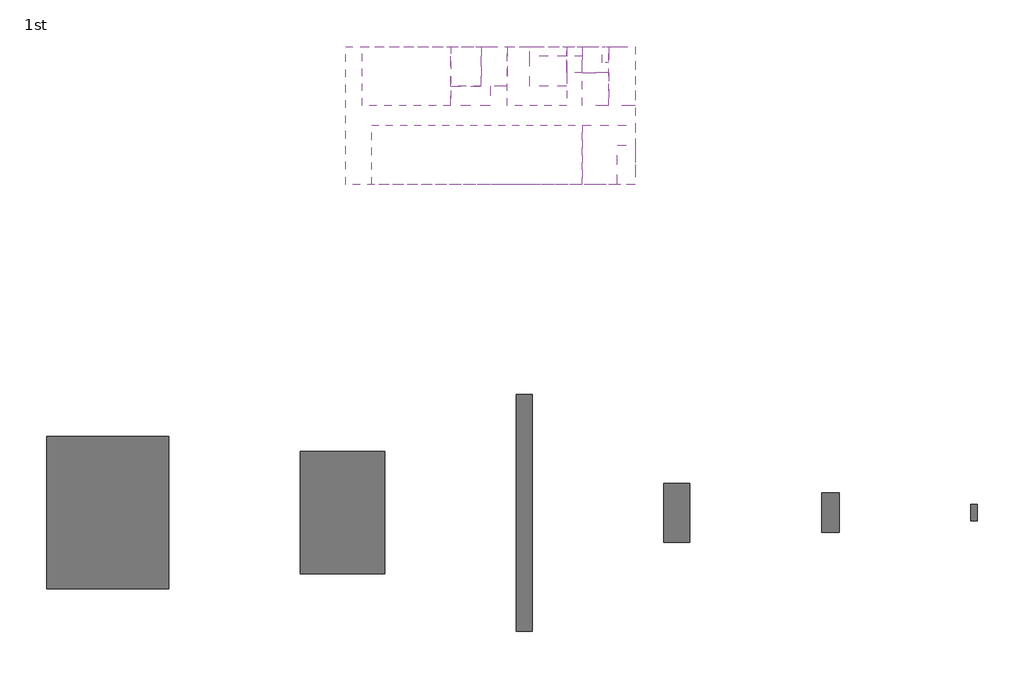
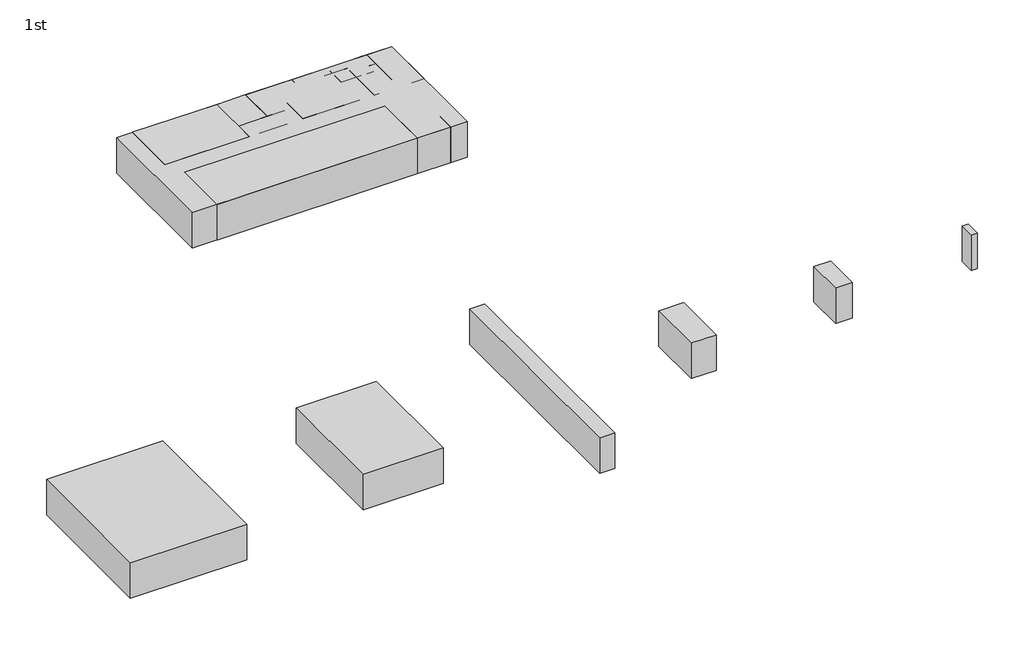
# One storey: 23 proxies.
"""IFC4 building model written with IfcOpenShell, lengths in millimetres."""

import ifcopenshell
import ifcopenshell.guid

model = None  # the IFC model being written
_history = None  # IfcOwnerHistory: only IFC2X3 demands one
_inside = {}  # id of a spatial element -> (the spatial element, [elements in it])
_under = {}  # id of a project, library or spatial element -> (it, [spatial elements below it])
_declared = {}  # id of a project -> (the project, [libraries it declares])
_typed = {}  # id of a type object -> (the type object, [elements of that type])
_made_of = {}  # id of a material, layer set ... -> (it, [elements and type objects made of it])


def new_model(schema):
    """Start an empty IFC model of exactly this schema.

    Asked for "IFC4X3", IfcOpenShell would pick the latest addendum, in which some entities
    have other attributes; the version numbers below select the first issue.
    IFC2X3 requires an IfcOwnerHistory on every rooted entity: one is made here for all.
    """
    global model, _history
    if schema == "IFC4X3":
        model = ifcopenshell.file(schema_version=(4, 3, 0, 0))
    else:
        model = ifcopenshell.file(schema=schema)
    _inside.clear()
    _under.clear()
    _declared.clear()
    _typed.clear()
    _made_of.clear()
    _history = None
    if model.schema == "IFC2X3":
        org = make("IfcOrganization", Name="unknown")
        user = make(
            "IfcPersonAndOrganization",
            ThePerson=make("IfcPerson", FamilyName="unknown"),
            TheOrganization=org,
        )
        app = make(
            "IfcApplication",
            ApplicationDeveloper=org,
            Version="unknown",
            ApplicationFullName="unknown",
            ApplicationIdentifier="unknown",
        )
        _history = make(
            "IfcOwnerHistory",
            OwningUser=user,
            OwningApplication=app,
            ChangeAction="ADDED",
            CreationDate=0,
        )
    return model


def make(cls, **values):
    """One entity of the class cls with the attributes given. An attribute that is None is left unset."""
    return model.create_entity(
        cls, **{name: value for name, value in values.items() if value is not None}
    )


def rooted(cls, **values):
    """An entity with a GlobalId (a new one), such as an element, a storey or a relation."""
    return make(cls, GlobalId=ifcopenshell.guid.new(), OwnerHistory=_history, **values)


def si_unit(unit_type, name, prefix=None):
    """IfcSIUnit, for example si_unit("LENGTHUNIT", "METRE", prefix="MILLI")."""
    return make("IfcSIUnit", UnitType=unit_type, Prefix=prefix, Name=name)


def assignment(units):
    """IfcUnitAssignment: the units of a project."""
    return None if units is None else make("IfcUnitAssignment", Units=units)


def point(xyz):
    """IfcCartesianPoint."""
    return None if xyz is None else make("IfcCartesianPoint", Coordinates=xyz)


def direction(xyz):
    """IfcDirection."""
    return None if xyz is None else make("IfcDirection", DirectionRatios=xyz)


def frame(location, z_axis=None, x_axis=None):
    """IfcAxis2Placement3D, a coordinate frame: its origin and axes. An axis left out is left unset."""
    return make(
        "IfcAxis2Placement3D",
        Location=point(location),
        Axis=direction(z_axis),
        RefDirection=direction(x_axis),
    )


def origin():
    """The frame at (0, 0, 0) with its axes left unset."""
    return frame((0.0, 0.0, 0.0))


def origin_with_axes():
    """The frame at (0, 0, 0) with the z axis (0, 0, 1) and the x axis (1, 0, 0) written out."""
    return frame((0.0, 0.0, 0.0), z_axis=(0.0, 0.0, 1.0), x_axis=(1.0, 0.0, 0.0))


def place(relative_to, where):
    """IfcLocalPlacement: puts the frame where relative to a parent placement (None: the world)."""
    return make(
        "IfcLocalPlacement", PlacementRelTo=relative_to, RelativePlacement=where
    )


def context(
    kind, dimensions, precision=None, world=None, true_north=None, identifier=None
):
    """IfcGeometricRepresentationContext, for example the 3D "Model" context."""
    return make(
        "IfcGeometricRepresentationContext",
        ContextIdentifier=identifier,
        ContextType=kind,
        CoordinateSpaceDimension=dimensions,
        Precision=precision,
        WorldCoordinateSystem=world,
        TrueNorth=true_north,
    )


def project(units=None, contexts=None):
    """IfcProject with its units and contexts."""
    return rooted(
        "IfcProject",
        Name="project",
        RepresentationContexts=contexts,
        UnitsInContext=assignment(units),
    )


def spatial(cls, under=None, at=None, **own):
    """A site, building, storey or space (cls), placed at a placement, below another one or the project."""
    s = rooted(cls, ObjectPlacement=at, **own)
    if under is not None:
        _under.setdefault(under.id(), (under, []))[1].append(s)
    return s


def polyline(points):
    """IfcPolyline through the points."""
    return make("IfcPolyline", Points=[point(p) for p in points])


def outline(outer, holes=None, kind="AREA"):
    """IfcArbitraryClosedProfileDef: a profile drawn as a closed curve; with holes, ...WithVoids."""
    if holes is None:
        return make("IfcArbitraryClosedProfileDef", ProfileType=kind, OuterCurve=outer)
    return make(
        "IfcArbitraryProfileDefWithVoids",
        ProfileType=kind,
        OuterCurve=outer,
        InnerCurves=holes,
    )


def extrude(swept, where, along, depth):
    """IfcExtrudedAreaSolid: the profile swept, set in the frame where, extruded along a direction by depth."""
    return make(
        "IfcExtrudedAreaSolid",
        SweptArea=swept,
        Position=where,
        ExtrudedDirection=direction(along),
        Depth=depth,
    )


def shape(context_of_items, identifier, shape_type, items):
    """IfcShapeRepresentation: the items that make up one representation, for example the "Body"."""
    return make(
        "IfcShapeRepresentation",
        ContextOfItems=context_of_items,
        RepresentationIdentifier=identifier,
        RepresentationType=shape_type,
        Items=items,
    )


def source(mapping_origin, context_of_items, identifier, shape_type, items):
    """IfcRepresentationMap: a shape defined once, which mapped items show again and again."""
    return make(
        "IfcRepresentationMap",
        MappingOrigin=mapping_origin,
        MappedRepresentation=shape(context_of_items, identifier, shape_type, items),
    )


def transform(
    local_origin,
    x_axis=None,
    y_axis=None,
    z_axis=None,
    scale=None,
    scale2=None,
    scale3=None,
    uniform=True,
):
    """IfcCartesianTransformationOperator3D, or its non-uniform kind. x_axis, y_axis, z_axis: its Axis1, 2, 3."""
    if uniform:
        return make(
            "IfcCartesianTransformationOperator3D",
            Axis1=direction(x_axis),
            Axis2=direction(y_axis),
            LocalOrigin=point(local_origin),
            Scale=scale,
            Axis3=direction(z_axis),
        )
    return make(
        "IfcCartesianTransformationOperator3DnonUniform",
        Axis1=direction(x_axis),
        Axis2=direction(y_axis),
        LocalOrigin=point(local_origin),
        Scale=scale,
        Axis3=direction(z_axis),
        Scale2=scale2,
        Scale3=scale3,
    )


def mapped(mapping_source, mapping_target):
    """IfcMappedItem: shows the shape of a source again, moved by a transform."""
    return make(
        "IfcMappedItem", MappingSource=mapping_source, MappingTarget=mapping_target
    )


def made_of(thing, what):
    """Note that an element or type object is made of a material, layer set ...; save() writes the relation."""
    if what is not None:
        _made_of.setdefault(what.id(), (what, []))[1].append(thing)
    return thing


def element(
    cls,
    number,
    at=None,
    inside=None,
    cuts=None,
    type_object=None,
    material=None,
    context=None,
    identifier="Body",
    shape_type=None,
    held_by="IfcProductDefinitionShape",
    body=None,
    shapes=None,
    **own,
):
    """One element of the class cls, such as IfcWall. Its Tag is "e" and its number.

    at: its placement. inside: the storey or other place that contains it. cuts: it is an
    opening in that element (IfcRelVoidsElement). A single representation is given by context,
    identifier, shape_type and body (its items); several are given by shapes. held_by: the class
    of the entity that holds the representations. save() writes the other relations.
    """
    e = rooted(cls, Tag="e%d" % number, ObjectPlacement=at, **own)
    if body is not None:
        shapes = [shape(context, identifier, shape_type, body)]
    if shapes is not None:
        e.Representation = make(held_by, Representations=shapes)
    if inside is not None:
        _inside.setdefault(inside.id(), (inside, []))[1].append(e)
    if cuts is not None:
        rooted(
            "IfcRelVoidsElement", RelatingBuildingElement=cuts, RelatedOpeningElement=e
        )
    if type_object is not None:
        _typed.setdefault(type_object.id(), (type_object, []))[1].append(e)
    return made_of(e, material)


def aggregate(whole, parts):
    """IfcRelAggregates: a whole, such as a stair, and the parts it consists of."""
    return rooted("IfcRelAggregates", RelatingObject=whole, RelatedObjects=parts)


def save(model, path):
    """Write the relations noted so far, then the file.

    IfcRelAggregates (storeys below a building ...), IfcRelContainedInSpatialStructure (elements
    in a storey), IfcRelDefinesByType, IfcRelAssociatesMaterial and IfcRelDeclares: one each for
    every whole, place, type object, material and project.
    """
    for whole, parts in _under.values():
        aggregate(whole, parts)
    for where, things in _inside.values():
        rooted(
            "IfcRelContainedInSpatialStructure",
            RelatedElements=things,
            RelatingStructure=where,
        )
    for kind, things in _typed.values():
        rooted("IfcRelDefinesByType", RelatedObjects=things, RelatingType=kind)
    for what, things in _made_of.values():
        rooted("IfcRelAssociatesMaterial", RelatedObjects=things, RelatingMaterial=what)
    for by, libraries in _declared.values():
        rooted("IfcRelDeclares", RelatingContext=by, RelatedDefinitions=libraries)
    model.write(path)


def generic_models_29bcd6f9(model_context):
    return source(origin(), model_context, "Body", "SweptSolid", [
        extrude(outline(polyline([(2000.0, 4500.0), (2000.0, -4500.0), (-2000.0, -4500.0), (-2000.0, 4500.0), (2000.0, 4500.0)])), origin_with_axes(), (0.0, 0.0, 1.0), 6000.0),
    ])


def generic_models_d82b1902(model_context):
    return source(origin(), model_context, "Body", "SweptSolid", [
        extrude(outline(polyline([(9300.0, 11600.0), (9300.0, -11600.0), (-9300.0, -11600.0), (-9300.0, 11600.0), (9300.0, 11600.0)])), origin_with_axes(), (0.0, 0.0, 1.0), 6000.0),
    ])


def generic_models_21711933(model_context):
    return source(origin(), model_context, "Body", "SweptSolid", [
        extrude(outline(polyline([(6400.0, 9300.0), (6400.0, -9300.0), (-6400.0, -9300.0), (-6400.0, 9300.0), (6400.0, 9300.0)])), origin_with_axes(), (0.0, 0.0, 1.0), 6000.0),
    ])


def generic_models_03d31222(model_context):
    return source(origin(), model_context, "Body", "SweptSolid", [
        extrude(outline(polyline([(1200.0, 18000.0), (1200.0, -18000.0), (-1200.0, -18000.0), (-1200.0, 18000.0), (1200.0, 18000.0)])), origin_with_axes(), (0.0, 0.0, 1.0), 6000.0),
    ])


def generic_models_5634f436(model_context):
    return source(origin(), model_context, "Body", "SweptSolid", [
        extrude(outline(polyline([(1350.0, 3000.0), (1350.0, -3000.0), (-1350.0, -3000.0), (-1350.0, 3000.0), (1350.0, 3000.0)])), origin_with_axes(), (0.0, 0.0, 1.0), 6000.0),
    ])


def generic_models_71e2440f(model_context):
    return source(origin(), model_context, "Body", "SweptSolid", [
        extrude(outline(polyline([(500.0, 1250.0), (500.0, -1250.0), (-500.0, -1250.0), (-500.0, 1250.0), (500.0, 1250.0)])), origin_with_axes(), (0.0, 0.0, 1.0), 6000.0),
    ])


def generic_models_57c7875f(model_context):
    return source(origin(), model_context, "Body", "SweptSolid", [
        extrude(outline(polyline([(4500.0, 16000.0), (4500.0, -16000.0), (-4500.0, -16000.0), (-4500.0, 16000.0), (4500.0, 16000.0)])), origin_with_axes(), (0.0, 0.0, 1.0), 6000.0),
    ])


def generic_models_7bff30ad(model_context):
    return source(origin(), model_context, "Body", "SweptSolid", [
        extrude(outline(polyline([(2000.0, 2000.0), (2000.0, -2000.0), (-2000.0, -2000.0), (-2000.0, 2000.0), (2000.0, 2000.0)])), origin_with_axes(), (0.0, 0.0, 1.0), 6000.0),
    ])


def generic_models_5b7b272c(model_context):
    return source(origin(), model_context, "Body", "SweptSolid", [
        extrude(outline(polyline([(2000.0, 2500.0), (2000.0, -2500.0), (-2000.0, -2500.0), (-2000.0, 2500.0), (2000.0, 2500.0)])), origin_with_axes(), (0.0, 0.0, 1.0), 6000.0),
    ])


def generic_models_47b98be1(model_context):
    return source(origin(), model_context, "Body", "SweptSolid", [
        extrude(outline(polyline([(1200.0, 2000.0), (1200.0, -2000.0), (-1200.0, -2000.0), (-1200.0, 2000.0), (1200.0, 2000.0)])), origin_with_axes(), (0.0, 0.0, 1.0), 6000.0),
    ])


def generic_models_7a053eeb(model_context):
    return source(origin(), model_context, "Body", "SweptSolid", [
        extrude(outline(polyline([(1200.0, 750.0), (1200.0, -750.0), (-1200.0, -750.0), (-1200.0, 750.0), (1200.0, 750.0)])), origin_with_axes(), (0.0, 0.0, 1.0), 6000.0),
    ])


def generic_models_ec17d728(model_context):
    return source(origin(), model_context, "Body", "SweptSolid", [
        extrude(outline(polyline([(2800.0, 3000.0), (2800.0, -3000.0), (-2800.0, -3000.0), (-2800.0, 3000.0), (2800.0, 3000.0)])), origin_with_axes(), (0.0, 0.0, 1.0), 6000.0),
    ])


def generic_models_85897e09(model_context):
    return source(origin(), model_context, "Body", "SweptSolid", [
        extrude(outline(polyline([(2800.0, 750.0), (2800.0, -750.0), (-2800.0, -750.0), (-2800.0, 750.0), (2800.0, 750.0)])), origin_with_axes(), (0.0, 0.0, 1.0), 6000.0),
    ])


def generic_models_b79df083(model_context):
    return source(origin(), model_context, "Body", "SweptSolid", [
        extrude(outline(polyline([(4500.0, 4500.0), (4500.0, -4500.0), (-4500.0, -4500.0), (-4500.0, 4500.0), (4500.0, 4500.0)])), origin_with_axes(), (0.0, 0.0, 1.0), 6000.0),
    ])


def generic_models_98b71764(model_context):
    return source(origin(), model_context, "Body", "SweptSolid", [
        extrude(outline(polyline([(2000.0, 3000.0), (2000.0, -3000.0), (-2000.0, -3000.0), (-2000.0, 3000.0), (2000.0, 3000.0)])), origin_with_axes(), (0.0, 0.0, 1.0), 6000.0),
    ])


def generic_models_1a87c0f4(model_context):
    return source(origin(), model_context, "Body", "SweptSolid", [
        extrude(outline(polyline([(2300.0, 3000.0), (2300.0, -3000.0), (-2300.0, -3000.0), (-2300.0, 3000.0), (2300.0, 3000.0)])), origin_with_axes(), (0.0, 0.0, 1.0), 6000.0),
    ])


def generic_models_df3bc381(model_context):
    return source(origin(), model_context, "Body", "SweptSolid", [
        extrude(outline(polyline([(4500.0, 6750.0), (4500.0, -6750.0), (-4500.0, -6750.0), (-4500.0, 6750.0), (4500.0, 6750.0)])), origin_with_axes(), (0.0, 0.0, 1.0), 6000.0),
    ])


def generic_models_542cc789(model_context):
    return source(origin(), model_context, "Body", "SweptSolid", [
        extrude(outline(polyline([(1500.0, 3000.0), (1500.0, -3000.0), (-1500.0, -3000.0), (-1500.0, 3000.0), (1500.0, 3000.0)])), origin_with_axes(), (0.0, 0.0, 1.0), 6000.0),
    ])


def generic_models_4d084078(model_context):
    return source(origin(), model_context, "Body", "SweptSolid", [
        extrude(outline(polyline([(4000.0, 4500.0), (4000.0, -4500.0), (-4000.0, -4500.0), (-4000.0, 4500.0), (4000.0, 4500.0)])), origin_with_axes(), (0.0, 0.0, 1.0), 6000.0),
    ])


def generic_models_7e8091d6(model_context):
    return source(origin(), model_context, "Body", "SweptSolid", [
        extrude(outline(polyline([(22000.0, 10500.0), (22000.0, -10500.0), (-22000.0, -10500.0), (-22000.0, 10500.0), (22000.0, 10500.0)])), origin_with_axes(), (0.0, 0.0, 1.0), 6000.0),
    ])


model = new_model("IFC4")

# Units and contexts
model_context = context("Model", 3, world=origin())
ifc_project = project(units=[si_unit("LENGTHUNIT", "METRE", prefix="MILLI")], contexts=[model_context])

# Site, building, storey
site = spatial("IfcSite", under=ifc_project)
building = spatial("IfcBuilding", under=site)
storey = spatial("IfcBuildingStorey", under=building, Name="1st", Elevation=6000.0)

# Proxies
placement = place(None, origin())
generic_models_shape = generic_models_29bcd6f9(model_context)
element("IfcBuildingElementProxy", 1, Name="Space Planning Box_hec : Space Planning Box_hec", ObjectType="Space Planning Box_hec : Space Planning Box_hec", at=placement, inside=storey, context=model_context, shape_type="MappedRepresentation", body=[
    mapped(generic_models_shape, transform((95800.0, 114000.0, 6000.0), x_axis=(1.0, 0.0, 0.0), y_axis=(0.0, 1.0, 0.0), z_axis=(0.0, 0.0, 1.0))),
])
element("IfcBuildingElementProxy", 2, Name="Space Planning Box_hec : Space Planning Box_hec", ObjectType="Space Planning Box_hec : Space Planning Box_hec", at=placement, inside=storey, context=model_context, shape_type="MappedRepresentation", body=[
    mapped(generic_models_shape, transform((87459.6521483, 180423.8614395, 12000.0), x_axis=(1.0, 0.0, 0.0), y_axis=(0.0, 1.0, 0.0), z_axis=(0.0, 0.0, 1.0))),
])
generic_models_2_shape = generic_models_d82b1902(model_context)
element("IfcBuildingElementProxy", 3, Name="Space Planning Box_hec : Space Planning Box_hec", ObjectType="Space Planning Box_hec : Space Planning Box_hec", at=placement, inside=storey, context=model_context, shape_type="MappedRepresentation", body=[
    mapped(generic_models_2_shape, transform((9300.0, 114000.0, 6000.0), x_axis=(1.0, 0.0, 0.0), y_axis=(0.0, 1.0, 0.0), z_axis=(0.0, 0.0, 1.0))),
])
generic_models_3_shape = generic_models_21711933(model_context)
element("IfcBuildingElementProxy", 4, Name="Space Planning Box_hec : Space Planning Box_hec", ObjectType="Space Planning Box_hec : Space Planning Box_hec", at=placement, inside=storey, context=model_context, shape_type="MappedRepresentation", body=[
    mapped(generic_models_3_shape, transform((45000.0, 114000.0, 6000.0), x_axis=(1.0, 0.0, 0.0), y_axis=(0.0, 1.0, 0.0), z_axis=(0.0, 0.0, 1.0))),
])
generic_models_4_shape = generic_models_03d31222(model_context)
element("IfcBuildingElementProxy", 5, Name="Space Planning Box_hec : Space Planning Box_hec", ObjectType="Space Planning Box_hec : Space Planning Box_hec", at=placement, inside=storey, context=model_context, shape_type="MappedRepresentation", body=[
    mapped(generic_models_4_shape, transform((72600.0, 114000.0, 6000.0), x_axis=(1.0, 0.0, 0.0), y_axis=(0.0, 1.0, 0.0), z_axis=(0.0, 0.0, 1.0))),
])
generic_models_5_shape = generic_models_5634f436(model_context)
element("IfcBuildingElementProxy", 6, Name="Space Planning Box_hec : Space Planning Box_hec", ObjectType="Space Planning Box_hec : Space Planning Box_hec", at=placement, inside=storey, context=model_context, shape_type="MappedRepresentation", body=[
    mapped(generic_models_5_shape, transform((119150.0, 114000.0, 6000.0), x_axis=(1.0, 0.0, 0.0), y_axis=(0.0, 1.0, 0.0), z_axis=(0.0, 0.0, 1.0))),
])
element("IfcBuildingElementProxy", 7, Name="Space Planning Box_hec : Space Planning Box_hec", ObjectType="Space Planning Box_hec : Space Planning Box_hec", at=placement, inside=storey, context=model_context, shape_type="MappedRepresentation", body=[
    mapped(generic_models_5_shape, transform((88109.6521483, 166923.8614395, 12000.0), x_axis=(1.0, 0.0, 0.0), y_axis=(0.0, 1.0, 0.0), z_axis=(0.0, 0.0, 1.0))),
])
generic_models_6_shape = generic_models_71e2440f(model_context)
element("IfcBuildingElementProxy", 8, Name="Space Planning Box_hec : Space Planning Box_hec", ObjectType="Space Planning Box_hec : Space Planning Box_hec", at=placement, inside=storey, context=model_context, shape_type="MappedRepresentation", body=[
    mapped(generic_models_6_shape, transform((141000.0, 114000.0, 6000.0), x_axis=(1.0, 0.0, 0.0), y_axis=(0.0, 1.0, 0.0), z_axis=(0.0, 0.0, 1.0))),
])
element("IfcBuildingElementProxy", 9, Name="Space Planning Box_hec : Space Planning Box_hec", ObjectType="Space Planning Box_hec : Space Planning Box_hec", at=placement, inside=storey, context=model_context, shape_type="MappedRepresentation", body=[
    mapped(generic_models_6_shape, transform((84959.6521483, 183673.8614395, 12000.0), x_axis=(1.0, 0.0, 0.0), y_axis=(0.0, 1.0, 0.0), z_axis=(0.0, 0.0, 1.0))),
])
generic_models_7_shape = generic_models_57c7875f(model_context)
element("IfcBuildingElementProxy", 10, Name="Space Planning Box_hec : Space Planning Box_hec", ObjectType="Space Planning Box_hec : Space Planning Box_hec", at=placement, inside=storey, context=model_context, shape_type="MappedRepresentation", body=[
    mapped(generic_models_7_shape, transform((65459.6521483, 168423.8614395, 12000.0), x_axis=(0.0, -1.0, 0.0), y_axis=(1.0, 0.0, 0.0), z_axis=(0.0, 0.0, 1.0))),
])
generic_models_8_shape = generic_models_7bff30ad(model_context)
element("IfcBuildingElementProxy", 11, Name="Space Planning Box_hec : Space Planning Box_hec", ObjectType="Space Planning Box_hec : Space Planning Box_hec", at=placement, inside=storey, context=model_context, shape_type="MappedRepresentation", body=[
    mapped(generic_models_8_shape, transform((83459.6521483, 182923.8614395, 12000.0), x_axis=(1.0, 0.0, 0.0), y_axis=(0.0, 1.0, 0.0), z_axis=(0.0, 0.0, 1.0))),
])
generic_models_9_shape = generic_models_5b7b272c(model_context)
element("IfcBuildingElementProxy", 12, Name="Space Planning Box_hec : Space Planning Box_hec", ObjectType="Space Planning Box_hec : Space Planning Box_hec", at=placement, inside=storey, context=model_context, shape_type="MappedRepresentation", body=[
    mapped(generic_models_9_shape, transform((83459.6521483, 178423.8614395, 12000.0), x_axis=(1.0, 0.0, 0.0), y_axis=(0.0, 1.0, 0.0), z_axis=(0.0, 0.0, 1.0))),
])
generic_models_10_shape = generic_models_47b98be1(model_context)
element("IfcBuildingElementProxy", 13, Name="Space Planning Box_hec : Space Planning Box_hec", ObjectType="Space Planning Box_hec : Space Planning Box_hec", at=placement, inside=storey, context=model_context, shape_type="MappedRepresentation", body=[
    mapped(generic_models_10_shape, transform((80259.6521483, 182923.8614395, 12000.0), x_axis=(1.0, 0.0, 0.0), y_axis=(0.0, 1.0, 0.0), z_axis=(0.0, 0.0, 1.0))),
])
generic_models_11_shape = generic_models_7a053eeb(model_context)
element("IfcBuildingElementProxy", 14, Name="Space Planning Box_hec : Space Planning Box_hec", ObjectType="Space Planning Box_hec : Space Planning Box_hec", at=placement, inside=storey, context=model_context, shape_type="MappedRepresentation", body=[
    mapped(generic_models_11_shape, transform((80259.6521483, 184173.8614395, 12000.0), x_axis=(1.0, 0.0, 0.0), y_axis=(0.0, 1.0, 0.0), z_axis=(0.0, 0.0, 1.0))),
])
generic_models_12_shape = generic_models_ec17d728(model_context)
element("IfcBuildingElementProxy", 15, Name="Space Planning Box_hec : Space Planning Box_hec", ObjectType="Space Planning Box_hec : Space Planning Box_hec", at=placement, inside=storey, context=model_context, shape_type="MappedRepresentation", body=[
    mapped(generic_models_12_shape, transform((76259.6521483, 181923.8614395, 12000.0), x_axis=(1.0, 0.0, 0.0), y_axis=(0.0, 1.0, 0.0), z_axis=(0.0, 0.0, 1.0))),
])
generic_models_13_shape = generic_models_85897e09(model_context)
element("IfcBuildingElementProxy", 16, Name="Space Planning Box_hec : Space Planning Box_hec", ObjectType="Space Planning Box_hec : Space Planning Box_hec", at=placement, inside=storey, context=model_context, shape_type="MappedRepresentation", body=[
    mapped(generic_models_13_shape, transform((76259.6521483, 184173.8614395, 12000.0), x_axis=(1.0, 0.0, 0.0), y_axis=(0.0, 1.0, 0.0), z_axis=(0.0, 0.0, 1.0))),
])
generic_models_14_shape = generic_models_b79df083(model_context)
element("IfcBuildingElementProxy", 17, Name="Space Planning Box_hec : Space Planning Box_hec", ObjectType="Space Planning Box_hec : Space Planning Box_hec", at=placement, inside=storey, context=model_context, shape_type="MappedRepresentation", body=[
    mapped(generic_models_14_shape, transform((74559.6521483, 180423.8614395, 12000.0), x_axis=(1.0, 0.0, 0.0), y_axis=(0.0, 1.0, 0.0), z_axis=(0.0, 0.0, 1.0))),
])
generic_models_15_shape = generic_models_98b71764(model_context)
element("IfcBuildingElementProxy", 18, Name="Space Planning Box_hec : Space Planning Box_hec", ObjectType="Space Planning Box_hec : Space Planning Box_hec", at=placement, inside=storey, context=model_context, shape_type="MappedRepresentation", body=[
    mapped(generic_models_15_shape, transform((68059.6521483, 181923.8614395, 12000.0), x_axis=(1.0, 0.0, 0.0), y_axis=(0.0, 1.0, 0.0), z_axis=(0.0, 0.0, 1.0))),
])
generic_models_16_shape = generic_models_1a87c0f4(model_context)
element("IfcBuildingElementProxy", 19, Name="Space Planning Box_hec : Space Planning Box_hec", ObjectType="Space Planning Box_hec : Space Planning Box_hec", at=placement, inside=storey, context=model_context, shape_type="MappedRepresentation", body=[
    mapped(generic_models_16_shape, transform((63759.6521483, 181923.8614395, 12000.0), x_axis=(1.0, 0.0, 0.0), y_axis=(0.0, 1.0, 0.0), z_axis=(0.0, 0.0, 1.0))),
])
generic_models_17_shape = generic_models_df3bc381(model_context)
element("IfcBuildingElementProxy", 20, Name="Space Planning Box_hec : Space Planning Box_hec", ObjectType="Space Planning Box_hec : Space Planning Box_hec", at=placement, inside=storey, context=model_context, shape_type="MappedRepresentation", body=[
    mapped(generic_models_17_shape, transform((54709.6521483, 180423.8614395, 12000.0), x_axis=(0.0, -1.0, 0.0), y_axis=(1.0, 0.0, 0.0), z_axis=(0.0, 0.0, 1.0))),
])
generic_models_18_shape = generic_models_542cc789(model_context)
element("IfcBuildingElementProxy", 21, Name="Space Planning Box_hec : Space Planning Box_hec", ObjectType="Space Planning Box_hec : Space Planning Box_hec", at=placement, inside=storey, context=model_context, shape_type="MappedRepresentation", body=[
    mapped(generic_models_18_shape, transform((64459.6521483, 177423.8614395, 12000.0), x_axis=(0.0, -1.0, 0.0), y_axis=(1.0, 0.0, 0.0), z_axis=(0.0, 0.0, 1.0))),
])
generic_models_19_shape = generic_models_4d084078(model_context)
element("IfcBuildingElementProxy", 22, Name="Space Planning Box_hec : Space Planning Box_hec", ObjectType="Space Planning Box_hec : Space Planning Box_hec", at=placement, inside=storey, context=model_context, shape_type="MappedRepresentation", body=[
    mapped(generic_models_19_shape, transform((85459.6521483, 168423.8614395, 12000.0), x_axis=(1.0, 0.0, 0.0), y_axis=(0.0, 1.0, 0.0), z_axis=(0.0, 0.0, 1.0))),
])
generic_models_20_shape = generic_models_7e8091d6(model_context)
element("IfcBuildingElementProxy", 23, Name="Space Planning Box_hec : Space Planning Box_hec", ObjectType="Space Planning Box_hec : Space Planning Box_hec", at=placement, inside=storey, context=model_context, shape_type="MappedRepresentation", body=[
    mapped(generic_models_20_shape, transform((67459.6521483, 174423.8614395, 12000.0), x_axis=(1.0, 0.0, 0.0), y_axis=(0.0, 1.0, 0.0), z_axis=(0.0, 0.0, 1.0))),
])

save(model, "model.ifc")

# Revit data of these elements
# Project information
#   Building Name = "MAIN GATE SECURITY BUILDING"
#   Project Status = "Project Status"
#   Client Name = "현대엔지니어링"
#   Project Address = "서울시 종로구 율곡로 75(계동)"
#   Project Name = "Therma Visayas Energy Project"
#   Project Number = "-"
# Grids (mm)
#   "A": line (45459.652, 190234.526) -> (45459.652, 152139.384)
#   "B": line (53459.652, 190234.526) -> (53459.652, 152139.384)
#   "C": line (61459.652, 190234.526) -> (61459.652, 152139.384)
#   "D": line (67459.652, 190234.526) -> (67459.652, 152139.384)
#   "E": line (73459.652, 190234.526) -> (73459.652, 152139.384)
#   "F": line (81459.652, 190234.526) -> (81459.652, 152139.384)
#   "G": line (85459.652, 190234.526) -> (85459.652, 152139.384)
#   "H": line (89459.652, 190234.526) -> (89459.652, 152139.384)
#   "4": line (39389.066, 184923.861) -> (102402.798, 184923.861)
#   "3": line (39389.066, 178923.861) -> (102402.798, 178923.861)
#   "2": line (39389.066, 172923.861) -> (102402.798, 172923.861)
#   "1": line (39389.066, 163923.861) -> (102402.798, 163923.861)
# Type "Space Planning Box_hec : Space Planning Box_hec"
#   Type Comments = "..."
#   Room Name [instance default] = "?"
#   Interior Finish [instance default] = ""
#   Exterior Finish [instance default] = ""
#   Department [instance default] = ""
#   Assembly Code = "..."
#   Width [instance default] = 1524 mm
#   Program Area [instance default] = 0.00 m²
#   Length [instance default] = 1524 mm
#   Height [instance default] = 1524 mm
#   Area [instance default] = 2.32258 m²
#   Fill Color [instance default] = Cyan
#   Default Elevation = 0
# Element 1 (IfcBuildingElementProxy, "Space Planning Box_hec : Space Planning Box_hec")
#   Room Name = "Stairway"
#   Interior Finish = "IF2"
#   Exterior Finish = "EF1"
#   Department = "AR"
#   Width = 4000 mm
#   Program Area = 36.00 m²
#   Length = 9000 mm
#   Height = 6000 mm
#   Area = 36.00 m²
#   Fill Color = Lavender
#   Phase Created = New Construction
#   Materials on its faces: "Lavender"
# Element 2 (IfcBuildingElementProxy, "Space Planning Box_hec : Space Planning Box_hec")
#   Room Name = "Stairway"
#   Interior Finish = "IF2"
#   Exterior Finish = "EF1"
#   Department = "AR"
#   Width = 4000 mm
#   Program Area = 38.00 m²
#   Length = 9000 mm
#   Height = 6000 mm
#   Area = 36.00 m²
#   Fill Color = Lavender
#   Phase Created = New Construction
#   Materials on its faces: "Lavender"
# Element 3 (IfcBuildingElementProxy, "Space Planning Box_hec : Space Planning Box_hec")
#   Room Name = "Electronic Room"
#   Interior Finish = "IF1"
#   Exterior Finish = "EF1"
#   Department = "CI"
#   Width = 18600 mm
#   Program Area = 431.52 m²
#   Length = 23200 mm
#   Height = 6000 mm
#   Area = 431.52 m²
#   Fill Color = Lime
#   Phase Created = New Construction
#   Materials on its faces: "Lime"
# Element 4 (IfcBuildingElementProxy, "Space Planning Box_hec : Space Planning Box_hec")
#   Room Name = "Electrical Room"
#   Interior Finish = "IF1"
#   Exterior Finish = "EF1"
#   Department = "EL"
#   Width = 12800 mm
#   Program Area = 238.08 m²
#   Length = 18600 mm
#   Height = 6000 mm
#   Area = 238.08 m²
#   Fill Color = Blue
#   Phase Created = New Construction
#   Materials on its faces: "Blue"
# Element 5 (IfcBuildingElementProxy, "Space Planning Box_hec : Space Planning Box_hec")
#   Room Name = "Corridor"
#   Interior Finish = "IF2-1"
#   Exterior Finish = "EF1"
#   Department = "AR"
#   Width = 2400 mm
#   Program Area = 86.40 m²
#   Length = 36000 mm
#   Height = 6000 mm
#   Area = 86.40 m²
#   Fill Color = Lavender
#   Phase Created = New Construction
#   Materials on its faces: "Lavender"
# Elements 6, 7 (IfcBuildingElementProxy, "Space Planning Box_hec : Space Planning Box_hec")
#   Room Name = "Duct Shaft"
#   Interior Finish = "NA"
#   Exterior Finish = "EF1"
#   Department = "HV"
#   Width = 2700 mm
#   Program Area = 16.20 m²
#   Length = 6000 mm
#   Height = 6000 mm
#   Area = 16.20 m²
#   Fill Color = Pink
#   Phase Created = New Construction
#   Materials on its faces: "Pink"
# Elements 8, 9 (IfcBuildingElementProxy, "Space Planning Box_hec : Space Planning Box_hec")
#   Room Name = "Pipe Shaft"
#   Interior Finish = "NA"
#   Exterior Finish = "EF1"
#   Department = "HV"
#   Width = 1000 mm
#   Program Area = 2.50 m²
#   Length = 2500 mm
#   Height = 6000 mm
#   Area = 2.50 m²
#   Fill Color = Pink
#   Phase Created = New Construction
#   Materials on its faces: "Pink"
# Element 10 (IfcBuildingElementProxy, "Space Planning Box_hec : Space Planning Box_hec")
#   Room Name = "Central Control Room"
#   Interior Finish = "IF3"
#   Exterior Finish = "EF1"
#   Department = "CI"
#   Width = 9000 mm
#   Program Area = 288.00 m²
#   Length = 32000 mm
#   Height = 6000 mm
#   Area = 288.00 m²
#   Fill Color = Lime
#   Phase Created = New Construction
#   Materials on its faces: "Lime"
# Element 11 (IfcBuildingElementProxy, "Space Planning Box_hec : Space Planning Box_hec")
#   Room Name = "Toilet (F)"
#   Interior Finish = "IF5"
#   Exterior Finish = "EF1"
#   Department = "AR"
#   Width = 4000 mm
#   Program Area = 72.00 m²
#   Length = 4000 mm
#   Height = 6000 mm
#   Area = 16.00 m²
#   Fill Color = Lavender
#   Phase Created = New Construction
#   Materials on its faces: "Lavender"
# Element 12 (IfcBuildingElementProxy, "Space Planning Box_hec : Space Planning Box_hec")
#   Room Name = "Toilet (M)"
#   Interior Finish = "IF5"
#   Exterior Finish = "EF1"
#   Department = "AR"
#   Width = 4000 mm
#   Program Area = 72.00 m²
#   Length = 5000 mm
#   Height = 6000 mm
#   Area = 20.00 m²
#   Fill Color = Lavender
#   Phase Created = New Construction
#   Materials on its faces: "Lavender"
# Element 13 (IfcBuildingElementProxy, "Space Planning Box_hec : Space Planning Box_hec")
#   Room Name = "Locker Room (F)"
#   Interior Finish = "IF2-1"
#   Exterior Finish = "EF1"
#   Department = "AR"
#   Width = 2400 mm
#   Program Area = 31.50 m²
#   Length = 4000 mm
#   Height = 6000 mm
#   Area = 9.60 m²
#   Fill Color = Lavender
#   Phase Created = New Construction
#   Materials on its faces: "Lavender"
# Element 14 (IfcBuildingElementProxy, "Space Planning Box_hec : Space Planning Box_hec")
#   Room Name = "Shower Room (F)"
#   Interior Finish = "IF5"
#   Exterior Finish = "EF1"
#   Department = "AR"
#   Width = 2400 mm
#   Program Area = 31.50 m²
#   Length = 1500 mm
#   Height = 6000 mm
#   Area = 3.60 m²
#   Fill Color = Lavender
#   Phase Created = New Construction
#   Materials on its faces: "Lavender"
# Element 15 (IfcBuildingElementProxy, "Space Planning Box_hec : Space Planning Box_hec")
#   Room Name = "Locker Room (M)"
#   Interior Finish = "IF2-1"
#   Exterior Finish = "EF1"
#   Department = "AR"
#   Width = 5600 mm
#   Program Area = 31.50 m²
#   Length = 6000 mm
#   Height = 6000 mm
#   Area = 33.60 m²
#   Fill Color = Lavender
#   Phase Created = New Construction
#   Materials on its faces: "Lavender"
# Element 16 (IfcBuildingElementProxy, "Space Planning Box_hec : Space Planning Box_hec")
#   Room Name = "Shower Room (M)"
#   Interior Finish = "IF5"
#   Exterior Finish = "EF1"
#   Department = "AR"
#   Width = 5600 mm
#   Program Area = 31.50 m²
#   Length = 1500 mm
#   Height = 6000 mm
#   Area = 8.40 m²
#   Fill Color = Lavender
#   Phase Created = New Construction
#   Materials on its faces: "Lavender"
# Element 17 (IfcBuildingElementProxy, "Space Planning Box_hec : Space Planning Box_hec")
#   Room Name = "Kitch & Lunch Room"
#   Interior Finish = "IF2-1"
#   Exterior Finish = "EF1"
#   Department = "AR"
#   Width = 9000 mm
#   Program Area = 31.50 m²
#   Length = 9000 mm
#   Height = 6000 mm
#   Area = 81.00 m²
#   Fill Color = Lavender
#   Phase Created = New Construction
#   Materials on its faces: "Lavender"
# Element 18 (IfcBuildingElementProxy, "Space Planning Box_hec : Space Planning Box_hec")
#   Room Name = "Shift Office Room"
#   Interior Finish = "IF2-1"
#   Exterior Finish = "EF1"
#   Department = "AR"
#   Width = 4000 mm
#   Program Area = 43.20 m²
#   Length = 6000 mm
#   Height = 6000 mm
#   Area = 24.00 m²
#   Fill Color = Lavender
#   Phase Created = New Construction
#   Materials on its faces: "Lavender"
# Element 19 (IfcBuildingElementProxy, "Space Planning Box_hec : Space Planning Box_hec")
#   Room Name = "Document Room"
#   Interior Finish = "IF2-1"
#   Exterior Finish = "EF1"
#   Department = "AR"
#   Width = 4600 mm
#   Program Area = 48.00 m²
#   Length = 6000 mm
#   Height = 6000 mm
#   Area = 27.60 m²
#   Fill Color = Lavender
#   Phase Created = New Construction
#   Materials on its faces: "Lavender"
# Element 20 (IfcBuildingElementProxy, "Space Planning Box_hec : Space Planning Box_hec")
#   Room Name = "Engineer Room"
#   Interior Finish = "IF3"
#   Exterior Finish = "EF1"
#   Department = "CI"
#   Width = 9000 mm
#   Program Area = 120.00 m²
#   Length = 13500 mm
#   Height = 6000 mm
#   Area = 121.50 m²
#   Fill Color = Lime
#   Phase Created = New Construction
#   Materials on its faces: "Lime"
# Element 21 (IfcBuildingElementProxy, "Space Planning Box_hec : Space Planning Box_hec")
#   Room Name = "LOTO Office Room"
#   Interior Finish = "IF2-1"
#   Exterior Finish = "EF1"
#   Department = "AR"
#   Width = 3000 mm
#   Program Area = 31.50 m²
#   Length = 6000 mm
#   Height = 6000 mm
#   Area = 18.00 m²
#   Fill Color = Lavender
#   Phase Created = New Construction
#   Materials on its faces: "Lavender"
# Element 22 (IfcBuildingElementProxy, "Space Planning Box_hec : Space Planning Box_hec")
#   Room Name = "Fire Gas Room"
#   Interior Finish = "IF1"
#   Exterior Finish = "EF1"
#   Department = "SF"
#   Width = 8000 mm
#   Program Area = 0.00 m²
#   Length = 9000 mm
#   Height = 6000 mm
#   Area = 72.00 m²
#   Fill Color = Cyan
#   Phase Created = New Construction
#   Materials on its faces: "Cyan"
# Element 23 (IfcBuildingElementProxy, "Space Planning Box_hec : Space Planning Box_hec")
#   Room Name = "Corridor"
#   Interior Finish = "IF2-1"
#   Exterior Finish = "EF1"
#   Department = "AR"
#   Width = 44000 mm
#   Program Area = 0.00 m²
#   Length = 21000 mm
#   Height = 6000 mm
#   Area = 924.00 m²
#   Fill Color = Lavender
#   Phase Created = New Construction
#   Materials on its faces: "Lavender"
# Materials
#   "Cyan": class "Generic", colour RGB 0 255 255, transparency 0.2, Cost = 0
#   "Lavender": class "Generic", colour RGB 186 85 211, transparency 0.2, Cost = 0
#   "Lime": class "Generic", colour RGB 0 255 0, transparency 0.2, Cost = 0
#   "Blue": class "Generic", colour RGB 0 0 255, transparency 0.2, Cost = 0
#   "Pink": class "Generic", colour RGB 255 105 180, transparency 0.2, Cost = 0
# Room at (65459.652, 168423.861) mm, phase "New Construction", upper offset 2438.4 mm, lower offset 0 mm
#   Number = "3.0"
#   Name = "a"
# Room at (54709.652, 180423.861) mm, phase "New Construction", upper offset 2438.4 mm, lower offset 0 mm
#   Number = "3.1"
#   Name = "a"
# Room at (63759.652, 181923.861) mm, phase "New Construction", upper offset 2438.4 mm, lower offset 0 mm
#   Number = "3.2"
#   Name = "a"
# Room at (83459.652, 178423.861) mm, phase "New Construction", upper offset 2438.4 mm, lower offset 0 mm
#   Number = "3.3"
#   Name = "a"
# Room at (87459.652, 180423.861) mm, phase "New Construction", upper offset 2438.4 mm, lower offset 0 mm
#   Number = "3.4"
#   Name = "a"
# Room at (68059.652, 181923.861) mm, phase "New Construction", upper offset 2438.4 mm, lower offset 0 mm
#   Number = "3.5"
#   Name = "a"
# Room at (64459.652, 177423.861) mm, phase "New Construction", upper offset 2438.4 mm, lower offset 0 mm
#   Number = "3.6"
#   Name = "a"
# Room at (80259.652, 184173.861) mm, phase "New Construction", upper offset 2438.4 mm, lower offset 0 mm
#   Number = "3.7"
#   Name = "a"
# Room at (67459.652, 174423.861) mm, phase "New Construction", upper offset 2438.4 mm, lower offset 0 mm
#   Number = "3.8"
#   Name = "a"
# Room at (80259.652, 182173.861) mm, phase "New Construction", upper offset 2438.4 mm, lower offset 0 mm
#   Number = "3.9"
#   Name = "a"
# Room at (76259.652, 184173.861) mm, phase "New Construction", upper offset 2438.4 mm, lower offset 0 mm
#   Number = "3.10"
#   Name = "a"
# Room at (74559.652, 178751.292) mm, phase "New Construction", upper offset 2438.4 mm, lower offset 0 mm
#   Number = "3.11"
#   Name = "a"
# Room at (76259.652, 181173.861) mm, phase "New Construction", upper offset 2438.4 mm, lower offset 0 mm
#   Number = "3.12"
#   Name = "a"
# Room at (85459.652, 168423.861) mm, phase "New Construction", upper offset 2438.4 mm, lower offset 0 mm
#   Number = "3.13"
#   Name = "a"
# Room at (88109.652, 166923.861) mm, phase "New Construction", upper offset 2438.4 mm, lower offset 0 mm
#   Number = "3.14"
#   Name = "a"
# Room at (83459.652, 182923.861) mm, phase "New Construction", upper offset 2438.4 mm, lower offset 0 mm
#   Number = "3.15"
#   Name = "a"
# Room at (84959.652, 183673.861) mm, phase "New Construction", upper offset 2438.4 mm, lower offset 0 mm
#   Number = "3.16"
#   Name = "a"
